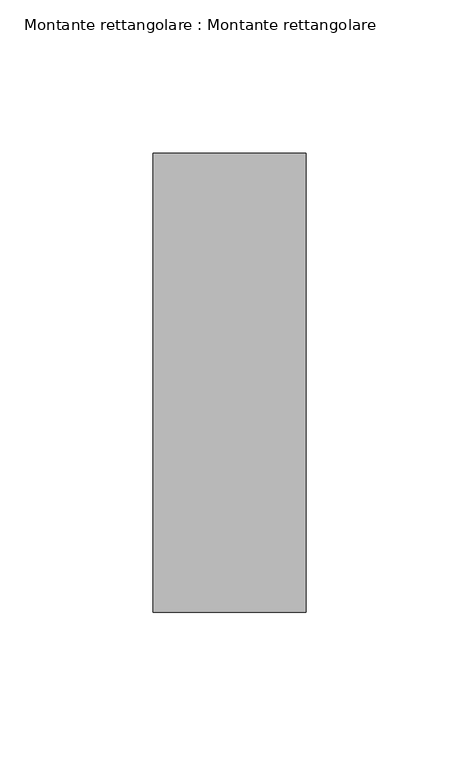
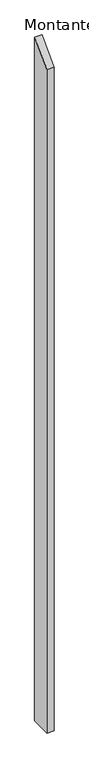
"""IFC4 building model written with IfcOpenShell, lengths in millimetres: member geometry, Montante rettangolare : Montante rettangolare."""

import ifcopenshell
import ifcopenshell.guid

model = None  # the IFC model being written
_history = None  # IfcOwnerHistory: only IFC2X3 demands one
_inside = {}  # id of a spatial element -> (the spatial element, [elements in it])
_under = {}  # id of a project, library or spatial element -> (it, [spatial elements below it])
_declared = {}  # id of a project -> (the project, [libraries it declares])
_typed = {}  # id of a type object -> (the type object, [elements of that type])
_made_of = {}  # id of a material, layer set ... -> (it, [elements and type objects made of it])


def new_model(schema):
    """Start an empty IFC model of exactly this schema.

    Asked for "IFC4X3", IfcOpenShell would pick the latest addendum, in which some entities
    have other attributes; the version numbers below select the first issue.
    IFC2X3 requires an IfcOwnerHistory on every rooted entity: one is made here for all.
    """
    global model, _history
    if schema == "IFC4X3":
        model = ifcopenshell.file(schema_version=(4, 3, 0, 0))
    else:
        model = ifcopenshell.file(schema=schema)
    _inside.clear()
    _under.clear()
    _declared.clear()
    _typed.clear()
    _made_of.clear()
    _history = None
    if model.schema == "IFC2X3":
        org = make("IfcOrganization", Name="unknown")
        user = make(
            "IfcPersonAndOrganization",
            ThePerson=make("IfcPerson", FamilyName="unknown"),
            TheOrganization=org,
        )
        app = make(
            "IfcApplication",
            ApplicationDeveloper=org,
            Version="unknown",
            ApplicationFullName="unknown",
            ApplicationIdentifier="unknown",
        )
        _history = make(
            "IfcOwnerHistory",
            OwningUser=user,
            OwningApplication=app,
            ChangeAction="ADDED",
            CreationDate=0,
        )
    return model


def make(cls, **values):
    """One entity of the class cls with the attributes given. An attribute that is None is left unset."""
    return model.create_entity(
        cls, **{name: value for name, value in values.items() if value is not None}
    )


def rooted(cls, **values):
    """An entity with a GlobalId (a new one), such as an element, a storey or a relation."""
    return make(cls, GlobalId=ifcopenshell.guid.new(), OwnerHistory=_history, **values)


def si_unit(unit_type, name, prefix=None):
    """IfcSIUnit, for example si_unit("LENGTHUNIT", "METRE", prefix="MILLI")."""
    return make("IfcSIUnit", UnitType=unit_type, Prefix=prefix, Name=name)


def assignment(units):
    """IfcUnitAssignment: the units of a project."""
    return None if units is None else make("IfcUnitAssignment", Units=units)


def point(xyz):
    """IfcCartesianPoint."""
    return None if xyz is None else make("IfcCartesianPoint", Coordinates=xyz)


def direction(xyz):
    """IfcDirection."""
    return None if xyz is None else make("IfcDirection", DirectionRatios=xyz)


def frame(location, z_axis=None, x_axis=None):
    """IfcAxis2Placement3D, a coordinate frame: its origin and axes. An axis left out is left unset."""
    return make(
        "IfcAxis2Placement3D",
        Location=point(location),
        Axis=direction(z_axis),
        RefDirection=direction(x_axis),
    )


def origin():
    """The frame at (0, 0, 0) with its axes left unset."""
    return frame((0.0, 0.0, 0.0))


def place(relative_to, where):
    """IfcLocalPlacement: puts the frame where relative to a parent placement (None: the world)."""
    return make(
        "IfcLocalPlacement", PlacementRelTo=relative_to, RelativePlacement=where
    )


def context(
    kind, dimensions, precision=None, world=None, true_north=None, identifier=None
):
    """IfcGeometricRepresentationContext, for example the 3D "Model" context."""
    return make(
        "IfcGeometricRepresentationContext",
        ContextIdentifier=identifier,
        ContextType=kind,
        CoordinateSpaceDimension=dimensions,
        Precision=precision,
        WorldCoordinateSystem=world,
        TrueNorth=true_north,
    )


def project(units=None, contexts=None):
    """IfcProject with its units and contexts."""
    return rooted(
        "IfcProject",
        Name="project",
        RepresentationContexts=contexts,
        UnitsInContext=assignment(units),
    )


def spatial(cls, under=None, at=None, **own):
    """A site, building, storey or space (cls), placed at a placement, below another one or the project."""
    s = rooted(cls, ObjectPlacement=at, **own)
    if under is not None:
        _under.setdefault(under.id(), (under, []))[1].append(s)
    return s


def polyline(points):
    """IfcPolyline through the points."""
    return make("IfcPolyline", Points=[point(p) for p in points])


def outline(outer, holes=None, kind="AREA"):
    """IfcArbitraryClosedProfileDef: a profile drawn as a closed curve; with holes, ...WithVoids."""
    if holes is None:
        return make("IfcArbitraryClosedProfileDef", ProfileType=kind, OuterCurve=outer)
    return make(
        "IfcArbitraryProfileDefWithVoids",
        ProfileType=kind,
        OuterCurve=outer,
        InnerCurves=holes,
    )


def extrude(swept, where, along, depth):
    """IfcExtrudedAreaSolid: the profile swept, set in the frame where, extruded along a direction by depth."""
    return make(
        "IfcExtrudedAreaSolid",
        SweptArea=swept,
        Position=where,
        ExtrudedDirection=direction(along),
        Depth=depth,
    )


def shape(context_of_items, identifier, shape_type, items):
    """IfcShapeRepresentation: the items that make up one representation, for example the "Body"."""
    return make(
        "IfcShapeRepresentation",
        ContextOfItems=context_of_items,
        RepresentationIdentifier=identifier,
        RepresentationType=shape_type,
        Items=items,
    )


def source(mapping_origin, context_of_items, identifier, shape_type, items):
    """IfcRepresentationMap: a shape defined once, which mapped items show again and again."""
    return make(
        "IfcRepresentationMap",
        MappingOrigin=mapping_origin,
        MappedRepresentation=shape(context_of_items, identifier, shape_type, items),
    )


def transform(
    local_origin,
    x_axis=None,
    y_axis=None,
    z_axis=None,
    scale=None,
    scale2=None,
    scale3=None,
    uniform=True,
):
    """IfcCartesianTransformationOperator3D, or its non-uniform kind. x_axis, y_axis, z_axis: its Axis1, 2, 3."""
    if uniform:
        return make(
            "IfcCartesianTransformationOperator3D",
            Axis1=direction(x_axis),
            Axis2=direction(y_axis),
            LocalOrigin=point(local_origin),
            Scale=scale,
            Axis3=direction(z_axis),
        )
    return make(
        "IfcCartesianTransformationOperator3DnonUniform",
        Axis1=direction(x_axis),
        Axis2=direction(y_axis),
        LocalOrigin=point(local_origin),
        Scale=scale,
        Axis3=direction(z_axis),
        Scale2=scale2,
        Scale3=scale3,
    )


def mapped(mapping_source, mapping_target):
    """IfcMappedItem: shows the shape of a source again, moved by a transform."""
    return make(
        "IfcMappedItem", MappingSource=mapping_source, MappingTarget=mapping_target
    )


def made_of(thing, what):
    """Note that an element or type object is made of a material, layer set ...; save() writes the relation."""
    if what is not None:
        _made_of.setdefault(what.id(), (what, []))[1].append(thing)
    return thing


def element(
    cls,
    number,
    at=None,
    inside=None,
    cuts=None,
    type_object=None,
    material=None,
    context=None,
    identifier="Body",
    shape_type=None,
    held_by="IfcProductDefinitionShape",
    body=None,
    shapes=None,
    **own,
):
    """One element of the class cls, such as IfcWall. Its Tag is "e" and its number.

    at: its placement. inside: the storey or other place that contains it. cuts: it is an
    opening in that element (IfcRelVoidsElement). A single representation is given by context,
    identifier, shape_type and body (its items); several are given by shapes. held_by: the class
    of the entity that holds the representations. save() writes the other relations.
    """
    e = rooted(cls, Tag="e%d" % number, ObjectPlacement=at, **own)
    if body is not None:
        shapes = [shape(context, identifier, shape_type, body)]
    if shapes is not None:
        e.Representation = make(held_by, Representations=shapes)
    if inside is not None:
        _inside.setdefault(inside.id(), (inside, []))[1].append(e)
    if cuts is not None:
        rooted(
            "IfcRelVoidsElement", RelatingBuildingElement=cuts, RelatedOpeningElement=e
        )
    if type_object is not None:
        _typed.setdefault(type_object.id(), (type_object, []))[1].append(e)
    return made_of(e, material)


def aggregate(whole, parts):
    """IfcRelAggregates: a whole, such as a stair, and the parts it consists of."""
    return rooted("IfcRelAggregates", RelatingObject=whole, RelatedObjects=parts)


def save(model, path):
    """Write the relations noted so far, then the file.

    IfcRelAggregates (storeys below a building ...), IfcRelContainedInSpatialStructure (elements
    in a storey), IfcRelDefinesByType, IfcRelAssociatesMaterial and IfcRelDeclares: one each for
    every whole, place, type object, material and project.
    """
    for whole, parts in _under.values():
        aggregate(whole, parts)
    for where, things in _inside.values():
        rooted(
            "IfcRelContainedInSpatialStructure",
            RelatedElements=things,
            RelatingStructure=where,
        )
    for kind, things in _typed.values():
        rooted("IfcRelDefinesByType", RelatedObjects=things, RelatingType=kind)
    for what, things in _made_of.values():
        rooted("IfcRelAssociatesMaterial", RelatedObjects=things, RelatingMaterial=what)
    for by, libraries in _declared.values():
        rooted("IfcRelDeclares", RelatingContext=by, RelatedDefinitions=libraries)
    model.write(path)


def montante_rettangolare_montante_rettangolare_44b40ab6(model_context):
    return source(origin(), model_context, "Body", "SweptSolid", [
        extrude(outline(polyline([(-75.0, -75.0), (75.0, 75.0), (75.0, -5005.0), (-75.0, -5005.0), (-75.0, -75.0)])), frame((-50.0, 0.0, 0.0), z_axis=(1.0, 0.0, 0.0), x_axis=(0.0, 1.0, 0.0)), (0.0, 0.0, 1.0), 50.0),
    ])


if __name__ == "__main__":
    model = new_model("IFC4")
    model_context = context("Model", 3, world=origin())
    ifc_project = project(units=[si_unit("LENGTHUNIT", "METRE", prefix="MILLI")], contexts=[model_context])
    site = spatial("IfcSite", under=ifc_project)
    building = spatial("IfcBuilding", under=site)
    placement = place(None, origin())
    montante_rettangolare_montante_rettangolare_shape = montante_rettangolare_montante_rettangolare_44b40ab6(model_context)
    element("IfcMember", 1, ObjectType="Montante rettangolare : Montante rettangolare", at=placement, inside=building, context=model_context, shape_type="MappedRepresentation", body=[
        mapped(montante_rettangolare_montante_rettangolare_shape, transform((0.0, 0.0, 0.0), x_axis=(1.0, 0.0, 0.0), y_axis=(0.0, 1.0, 0.0), z_axis=(0.0, 0.0, 1.0))),
    ])
    save(model, "model.ifc")

# Revit data of these elements
# Type "Montante rettangolare : Montante rettangolare"
#   built-in parameter 1007304 = 0.492126 (stored number, unit not read)
#   built-in parameter 1007301 = 0.082021 (stored number, unit not read)
#   built-in parameter 1007300 = 0.082021 (stored number, unit not read)
# Element 1 (IfcMember, "Montante rettangolare : Montante rettangolare")
#   Materials on its faces: "Acciaio"
# Materials
#   "Acciaio": class "Metallo", colour RGB 247 247 247, transparency 0, Description = "Acciaio, finitura zigrinata", Cost = 0
